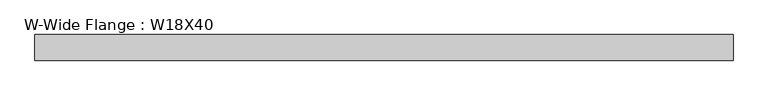
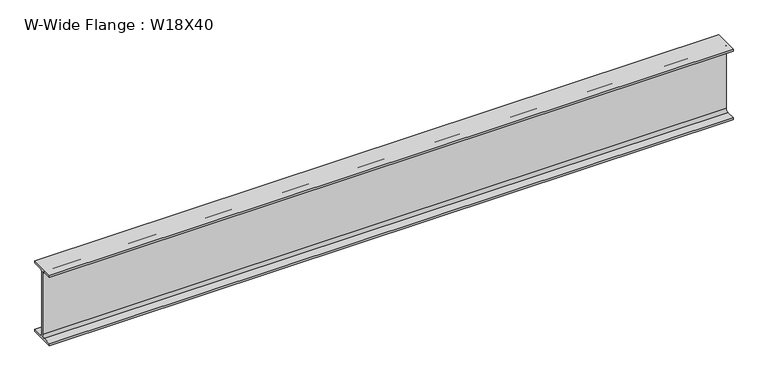
"""IFC4 building model written with IfcOpenShell, lengths in millimetres: beam geometry, W-Wide Flange : W18X40."""

from ifc_helpers import new_model, si_unit, point, frame, frame_2d, origin, place, context, project, spatial, polyline, circle_curve, trimmed, segment, composite_curve, outline, extrude, source, transform, mapped, element, save


def w_wide_flange_w18x40_a0ae42b6(model_context):
    return source(origin(), model_context, "Body", "SweptSolid", [
        extrude(outline(composite_curve([segment(polyline([(76.454, -213.995), (76.454, -227.33), (-76.454, -227.33), (-76.454, -213.995), (-20.828, -213.995)]), True, "CONTINUOUS"), segment(trimmed(circle_curve(frame_2d((-20.828, -197.1675)), 16.8275), [point((-20.828, -213.995))], [point((-4.0005, -197.1675))], True, "CARTESIAN"), True, "CONTINUOUS"), segment(polyline([(-4.0005, -197.1675), (-4.0005, 197.1675)]), True, "CONTINUOUS"), segment(trimmed(circle_curve(frame_2d((-20.828, 197.1675)), 16.8275), [point((-4.0005, 197.1675))], [point((-20.828, 213.995))], True, "CARTESIAN"), True, "CONTINUOUS"), segment(polyline([(-20.828, 213.995), (-76.454, 213.995), (-76.454, 227.33), (76.454, 227.33), (76.454, 213.995), (20.828, 213.995)]), True, "CONTINUOUS"), segment(trimmed(circle_curve(frame_2d((20.828, 197.1675)), 16.8275), [point((20.828, 213.995))], [point((4.0005, 197.1675))], True, "CARTESIAN"), True, "CONTINUOUS"), segment(polyline([(4.0005, 197.1675), (4.0005, -197.1675)]), True, "CONTINUOUS"), segment(trimmed(circle_curve(frame_2d((20.828, -197.1675)), 16.8275), [point((4.0005, -197.1675))], [point((20.828, -213.995))], True, "CARTESIAN"), True, "CONTINUOUS"), segment(polyline([(20.828, -213.995), (76.454, -213.995)]), True, "CONTINUOUS")], self_intersect=False)), frame((-2082.8, 0.0, 0.0), z_axis=(1.0, 0.0, 0.0), x_axis=(0.0, 1.0, 0.0)), (0.0, 0.0, 1.0), 4165.6),
    ])


if __name__ == "__main__":
    model = new_model("IFC4")
    model_context = context("Model", 3, world=origin())
    ifc_project = project(units=[si_unit("LENGTHUNIT", "METRE", prefix="MILLI")], contexts=[model_context])
    site = spatial("IfcSite", under=ifc_project)
    building = spatial("IfcBuilding", under=site)
    placement = place(None, origin())
    w_wide_flange_w18x40_shape = w_wide_flange_w18x40_a0ae42b6(model_context)
    element("IfcBeam", 1, ObjectType="W-Wide Flange : W18X40", at=placement, inside=building, context=model_context, shape_type="MappedRepresentation", body=[
        mapped(w_wide_flange_w18x40_shape, transform((0.0, 0.0, 0.0), x_axis=(1.0, 0.0, 0.0), y_axis=(0.0, 1.0, 0.0), z_axis=(0.0, 0.0, 1.0))),
    ])
    save(model, "model.ifc")

# Revit data of these elements
# Type "W-Wide Flange : W18X40"
#   Assembly Code = "B10"
#   W = 40
#   Length [instance default] = 5' - 0"
#   bf = 0' - 6.02"
#   d = 1' - 5.9"
#   k = 0' - 1 3/16"
#   k2 = 0' - 0.6625"
#   tf = 0' - 0.525"
#   tw = 0' - 0.315"
#   A = 0.0819444 SF
#   Structural Material [instance default] = Steel ASTM A992
# Element 1 (IfcBeam, "W-Wide Flange : W18X40")
#   Materials on its faces: "Steel ASTM A992"
# Materials
#   "Steel ASTM A992": class "Metal", colour RGB 199 199 199, transparency 0, Description = "Structural steel 50ksi", Cost = 0
